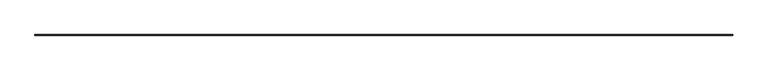
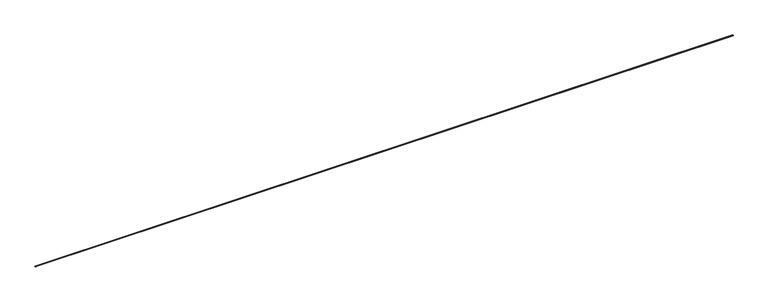
"""IFC4 building model written with IfcOpenShell, lengths in millimetres: proxy geometry, Inner panel:Inner panel:1:Inner panel:1 : Inner panel:Inner panel:300324:2:Inner panel:1:Inner panel:1 : Inner panel:Inner panel:300324:2 : Inner panel:Inner panel:1:Inner panel:1 : Inner panel:Inner panel:300324:300043:26 : Inner panel:Inner panel:1:Inner panel:1 : Inner panel:Inner panel:300324:2:Inner panel:1:Inner panel:1 : Inner panel:Inner panel:300324:2 : Inner panel:Inner panel:1:Inner panel:1 : Inner panel:Inner panel:300324:300043:308120."""

import ifcopenshell
import ifcopenshell.guid

model = None  # the IFC model being written
_history = None  # IfcOwnerHistory: only IFC2X3 demands one
_inside = {}  # id of a spatial element -> (the spatial element, [elements in it])
_under = {}  # id of a project, library or spatial element -> (it, [spatial elements below it])
_declared = {}  # id of a project -> (the project, [libraries it declares])
_typed = {}  # id of a type object -> (the type object, [elements of that type])
_made_of = {}  # id of a material, layer set ... -> (it, [elements and type objects made of it])


def new_model(schema):
    """Start an empty IFC model of exactly this schema.

    Asked for "IFC4X3", IfcOpenShell would pick the latest addendum, in which some entities
    have other attributes; the version numbers below select the first issue.
    IFC2X3 requires an IfcOwnerHistory on every rooted entity: one is made here for all.
    """
    global model, _history
    if schema == "IFC4X3":
        model = ifcopenshell.file(schema_version=(4, 3, 0, 0))
    else:
        model = ifcopenshell.file(schema=schema)
    _inside.clear()
    _under.clear()
    _declared.clear()
    _typed.clear()
    _made_of.clear()
    _history = None
    if model.schema == "IFC2X3":
        org = make("IfcOrganization", Name="unknown")
        user = make(
            "IfcPersonAndOrganization",
            ThePerson=make("IfcPerson", FamilyName="unknown"),
            TheOrganization=org,
        )
        app = make(
            "IfcApplication",
            ApplicationDeveloper=org,
            Version="unknown",
            ApplicationFullName="unknown",
            ApplicationIdentifier="unknown",
        )
        _history = make(
            "IfcOwnerHistory",
            OwningUser=user,
            OwningApplication=app,
            ChangeAction="ADDED",
            CreationDate=0,
        )
    return model


def make(cls, **values):
    """One entity of the class cls with the attributes given. An attribute that is None is left unset."""
    return model.create_entity(
        cls, **{name: value for name, value in values.items() if value is not None}
    )


def rooted(cls, **values):
    """An entity with a GlobalId (a new one), such as an element, a storey or a relation."""
    return make(cls, GlobalId=ifcopenshell.guid.new(), OwnerHistory=_history, **values)


def si_unit(unit_type, name, prefix=None):
    """IfcSIUnit, for example si_unit("LENGTHUNIT", "METRE", prefix="MILLI")."""
    return make("IfcSIUnit", UnitType=unit_type, Prefix=prefix, Name=name)


def assignment(units):
    """IfcUnitAssignment: the units of a project."""
    return None if units is None else make("IfcUnitAssignment", Units=units)


def point(xyz):
    """IfcCartesianPoint."""
    return None if xyz is None else make("IfcCartesianPoint", Coordinates=xyz)


def direction(xyz):
    """IfcDirection."""
    return None if xyz is None else make("IfcDirection", DirectionRatios=xyz)


def frame(location, z_axis=None, x_axis=None):
    """IfcAxis2Placement3D, a coordinate frame: its origin and axes. An axis left out is left unset."""
    return make(
        "IfcAxis2Placement3D",
        Location=point(location),
        Axis=direction(z_axis),
        RefDirection=direction(x_axis),
    )


def origin():
    """The frame at (0, 0, 0) with its axes left unset."""
    return frame((0.0, 0.0, 0.0))


def place(relative_to, where):
    """IfcLocalPlacement: puts the frame where relative to a parent placement (None: the world)."""
    return make(
        "IfcLocalPlacement", PlacementRelTo=relative_to, RelativePlacement=where
    )


def context(
    kind, dimensions, precision=None, world=None, true_north=None, identifier=None
):
    """IfcGeometricRepresentationContext, for example the 3D "Model" context."""
    return make(
        "IfcGeometricRepresentationContext",
        ContextIdentifier=identifier,
        ContextType=kind,
        CoordinateSpaceDimension=dimensions,
        Precision=precision,
        WorldCoordinateSystem=world,
        TrueNorth=true_north,
    )


def project(units=None, contexts=None):
    """IfcProject with its units and contexts."""
    return rooted(
        "IfcProject",
        Name="project",
        RepresentationContexts=contexts,
        UnitsInContext=assignment(units),
    )


def spatial(cls, under=None, at=None, **own):
    """A site, building, storey or space (cls), placed at a placement, below another one or the project."""
    s = rooted(cls, ObjectPlacement=at, **own)
    if under is not None:
        _under.setdefault(under.id(), (under, []))[1].append(s)
    return s


def polyline(points):
    """IfcPolyline through the points."""
    return make("IfcPolyline", Points=[point(p) for p in points])


def outline(outer, holes=None, kind="AREA"):
    """IfcArbitraryClosedProfileDef: a profile drawn as a closed curve; with holes, ...WithVoids."""
    if holes is None:
        return make("IfcArbitraryClosedProfileDef", ProfileType=kind, OuterCurve=outer)
    return make(
        "IfcArbitraryProfileDefWithVoids",
        ProfileType=kind,
        OuterCurve=outer,
        InnerCurves=holes,
    )


def extrude(swept, where, along, depth):
    """IfcExtrudedAreaSolid: the profile swept, set in the frame where, extruded along a direction by depth."""
    return make(
        "IfcExtrudedAreaSolid",
        SweptArea=swept,
        Position=where,
        ExtrudedDirection=direction(along),
        Depth=depth,
    )


def shape(context_of_items, identifier, shape_type, items):
    """IfcShapeRepresentation: the items that make up one representation, for example the "Body"."""
    return make(
        "IfcShapeRepresentation",
        ContextOfItems=context_of_items,
        RepresentationIdentifier=identifier,
        RepresentationType=shape_type,
        Items=items,
    )


def source(mapping_origin, context_of_items, identifier, shape_type, items):
    """IfcRepresentationMap: a shape defined once, which mapped items show again and again."""
    return make(
        "IfcRepresentationMap",
        MappingOrigin=mapping_origin,
        MappedRepresentation=shape(context_of_items, identifier, shape_type, items),
    )


def transform(
    local_origin,
    x_axis=None,
    y_axis=None,
    z_axis=None,
    scale=None,
    scale2=None,
    scale3=None,
    uniform=True,
):
    """IfcCartesianTransformationOperator3D, or its non-uniform kind. x_axis, y_axis, z_axis: its Axis1, 2, 3."""
    if uniform:
        return make(
            "IfcCartesianTransformationOperator3D",
            Axis1=direction(x_axis),
            Axis2=direction(y_axis),
            LocalOrigin=point(local_origin),
            Scale=scale,
            Axis3=direction(z_axis),
        )
    return make(
        "IfcCartesianTransformationOperator3DnonUniform",
        Axis1=direction(x_axis),
        Axis2=direction(y_axis),
        LocalOrigin=point(local_origin),
        Scale=scale,
        Axis3=direction(z_axis),
        Scale2=scale2,
        Scale3=scale3,
    )


def mapped(mapping_source, mapping_target):
    """IfcMappedItem: shows the shape of a source again, moved by a transform."""
    return make(
        "IfcMappedItem", MappingSource=mapping_source, MappingTarget=mapping_target
    )


def made_of(thing, what):
    """Note that an element or type object is made of a material, layer set ...; save() writes the relation."""
    if what is not None:
        _made_of.setdefault(what.id(), (what, []))[1].append(thing)
    return thing


def element(
    cls,
    number,
    at=None,
    inside=None,
    cuts=None,
    type_object=None,
    material=None,
    context=None,
    identifier="Body",
    shape_type=None,
    held_by="IfcProductDefinitionShape",
    body=None,
    shapes=None,
    **own,
):
    """One element of the class cls, such as IfcWall. Its Tag is "e" and its number.

    at: its placement. inside: the storey or other place that contains it. cuts: it is an
    opening in that element (IfcRelVoidsElement). A single representation is given by context,
    identifier, shape_type and body (its items); several are given by shapes. held_by: the class
    of the entity that holds the representations. save() writes the other relations.
    """
    e = rooted(cls, Tag="e%d" % number, ObjectPlacement=at, **own)
    if body is not None:
        shapes = [shape(context, identifier, shape_type, body)]
    if shapes is not None:
        e.Representation = make(held_by, Representations=shapes)
    if inside is not None:
        _inside.setdefault(inside.id(), (inside, []))[1].append(e)
    if cuts is not None:
        rooted(
            "IfcRelVoidsElement", RelatingBuildingElement=cuts, RelatedOpeningElement=e
        )
    if type_object is not None:
        _typed.setdefault(type_object.id(), (type_object, []))[1].append(e)
    return made_of(e, material)


def aggregate(whole, parts):
    """IfcRelAggregates: a whole, such as a stair, and the parts it consists of."""
    return rooted("IfcRelAggregates", RelatingObject=whole, RelatedObjects=parts)


def save(model, path):
    """Write the relations noted so far, then the file.

    IfcRelAggregates (storeys below a building ...), IfcRelContainedInSpatialStructure (elements
    in a storey), IfcRelDefinesByType, IfcRelAssociatesMaterial and IfcRelDeclares: one each for
    every whole, place, type object, material and project.
    """
    for whole, parts in _under.values():
        aggregate(whole, parts)
    for where, things in _inside.values():
        rooted(
            "IfcRelContainedInSpatialStructure",
            RelatedElements=things,
            RelatingStructure=where,
        )
    for kind, things in _typed.values():
        rooted("IfcRelDefinesByType", RelatedObjects=things, RelatingType=kind)
    for what, things in _made_of.values():
        rooted("IfcRelAssociatesMaterial", RelatedObjects=things, RelatingMaterial=what)
    for by, libraries in _declared.values():
        rooted("IfcRelDeclares", RelatingContext=by, RelatedDefinitions=libraries)
    model.write(path)


def generic_models_bcfb0a8f(model_context):
    return source(origin(), model_context, "Body", "SweptSolid", [
        extrude(outline(polyline([(-576538.5932007, 4014.3527172), (-576540.1132359, 4050.8335635), (-576582.9913922, 4049.0469737), (-576581.471357, 4012.5661273), (-576598.145764, 4011.8713604), (-576598.3030045, 4015.6451333), (-576596.7141271, 4015.6451333), (-576596.6257287, 4013.5235726), (-576583.1235692, 4014.0861626), (-576584.6436045, 4050.5670089), (-576538.5932007, 4052.4857758), (-576537.0731654, 4016.0049294), (-576523.5710059, 4016.5675194), (-576523.662158, 4018.7551686), (-576522.0732805, 4018.7551686), (-576521.9187937, 4015.0474841), (-576538.5932007, 4014.3527172)])), frame((579104.5117239, 0.0, 0.0), z_axis=(1.0, 0.0, 0.0), x_axis=(0.0, 1.0, 0.0)), (0.0, 0.0, 1.0), 88442.8),
    ])


if __name__ == "__main__":
    model = new_model("IFC4")
    model_context = context("Model", 3, world=origin())
    ifc_project = project(units=[si_unit("LENGTHUNIT", "METRE", prefix="MILLI")], contexts=[model_context])
    site = spatial("IfcSite", under=ifc_project)
    building = spatial("IfcBuilding", under=site)
    placement = place(None, origin())
    generic_models_shape = generic_models_bcfb0a8f(model_context)
    element("IfcBuildingElementProxy", 1, Name="Inner panel:Inner panel:1:Inner panel:1 : Inner panel:Inner panel:300324:2:Inner panel:1:Inner panel:1 : Inner panel:Inner panel:300324:2 : Inner panel:Inner panel:1:Inner panel:1 : Inner panel:Inner panel:300324:300043:26 : Inner panel:Inner panel:1:Inner panel:1 : Inner panel:Inner panel:300324:2:Inner panel:1:Inner panel:1 : Inner panel:Inner panel:300324:2 : Inner panel:Inner panel:1:Inner panel:1 : Inner panel:Inner panel:300324:300043:308120", ObjectType="Inner panel:Inner panel:1:Inner panel:1 : Inner panel:Inner panel:300324:2:Inner panel:1:Inner panel:1 : Inner panel:Inner panel:300324:2 : Inner panel:Inner panel:1:Inner panel:1 : Inner panel:Inner panel:300324:300043:26 : Inner panel:Inner panel:1:Inner panel:1 : Inner panel:Inner panel:300324:2:Inner panel:1:Inner panel:1 : Inner panel:Inner panel:300324:2 : Inner panel:Inner panel:1:Inner panel:1 : Inner panel:Inner panel:300324:300043:308120", at=placement, inside=building, context=model_context, shape_type="MappedRepresentation", body=[
        mapped(generic_models_shape, transform((0.0, 0.0, 0.0), x_axis=(1.0, 0.0, 0.0), y_axis=(0.0, 1.0, 0.0), z_axis=(0.0, 0.0, 1.0))),
    ])
    save(model, "model.ifc")

# Revit data of these elements
# Type "Inner panel:Inner panel:1:Inner panel:1 : Inner panel:Inner panel:300324:2:Inner panel:1:Inner panel:1 : Inner panel:Inner panel:300324:2 : Inner panel:Inner panel:1:Inner panel:1 : Inner panel:Inner panel:300324:300043:26 : Inner panel:Inner panel:1:Inner panel:1 : Inner panel:Inner panel:300324:2:Inner panel:1:Inner panel:1 : Inner panel:Inner panel:300324:2 : Inner panel:Inner panel:1:Inner panel:1 : Inner panel:Inner panel:300324:300043:308120"
#   NameOverride = "Inner panel:Inner panel:1:Inner panel:1 : Inner panel:Inner panel:300324:2:Inner panel:1:Inner panel:1 : Inner panel:Inner panel:300324:2 : Inner panel:Inner panel:1:Inner panel:1 : Inner panel:Inner panel:300324:300043:308120"
#   ObjectTypeOverride = "Inner panel:1:Inner panel:1 : Inner panel:Inner panel:300324:2 : Inner panel:Inner panel:1:Inner panel:1 : Inner panel:Inner panel:300324:300043"
#   Reference = "Inner panel"
#   Tag = "308120"
# Element 1 (IfcBuildingElementProxy, "Inner panel:Inner panel:1:Inner panel:1 : Inner panel:Inner panel:300324:2:Inner panel:1:Inner panel:1 : Inner panel:Inner panel:300324:2 : Inner panel:Inner panel:1:Inner panel:1 : Inner panel:Inner panel:300324:300043:26 : Inner panel:Inner panel:1:Inner panel:1 : Inner panel:Inner panel:300324:2:Inner panel:1:Inner panel:1 : Inner panel:Inner panel:300324:2 : Inner panel:Inner panel:1:Inner panel:1 : Inner panel:Inner panel:300324:300043:308120")
#   Materials on its faces: "1 1/2\" HAT CHANNELS - SEE STRUCT. DWGs"
# Materials
#   "1 1/2\" HAT CHANNELS - SEE STRUCT. DWGs": class "Metal", colour RGB 189 187 185, transparency 0, Description = "Structural steel 50ksi", Cost = 0
